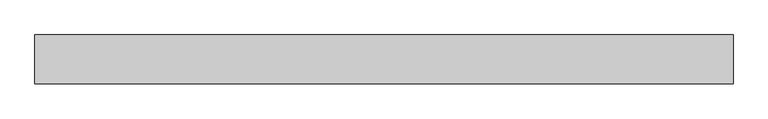
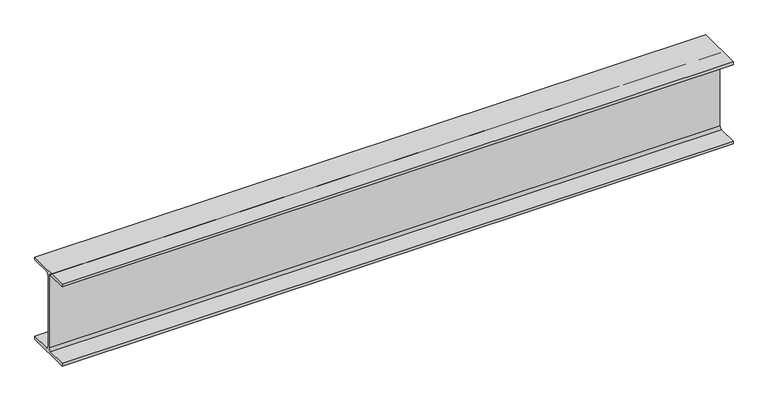
"""IFC4 building model written with IfcOpenShell, lengths in millimetres: beam geometry, Old_Steel Beam_H-KSD3502 : H_SB_ASB_H-200×200x8x12."""

import ifcopenshell
import ifcopenshell.guid

model = None  # the IFC model being written
_history = None  # IfcOwnerHistory: only IFC2X3 demands one
_inside = {}  # id of a spatial element -> (the spatial element, [elements in it])
_under = {}  # id of a project, library or spatial element -> (it, [spatial elements below it])
_declared = {}  # id of a project -> (the project, [libraries it declares])
_typed = {}  # id of a type object -> (the type object, [elements of that type])
_made_of = {}  # id of a material, layer set ... -> (it, [elements and type objects made of it])


def new_model(schema):
    """Start an empty IFC model of exactly this schema.

    Asked for "IFC4X3", IfcOpenShell would pick the latest addendum, in which some entities
    have other attributes; the version numbers below select the first issue.
    IFC2X3 requires an IfcOwnerHistory on every rooted entity: one is made here for all.
    """
    global model, _history
    if schema == "IFC4X3":
        model = ifcopenshell.file(schema_version=(4, 3, 0, 0))
    else:
        model = ifcopenshell.file(schema=schema)
    _inside.clear()
    _under.clear()
    _declared.clear()
    _typed.clear()
    _made_of.clear()
    _history = None
    if model.schema == "IFC2X3":
        org = make("IfcOrganization", Name="unknown")
        user = make(
            "IfcPersonAndOrganization",
            ThePerson=make("IfcPerson", FamilyName="unknown"),
            TheOrganization=org,
        )
        app = make(
            "IfcApplication",
            ApplicationDeveloper=org,
            Version="unknown",
            ApplicationFullName="unknown",
            ApplicationIdentifier="unknown",
        )
        _history = make(
            "IfcOwnerHistory",
            OwningUser=user,
            OwningApplication=app,
            ChangeAction="ADDED",
            CreationDate=0,
        )
    return model


def make(cls, **values):
    """One entity of the class cls with the attributes given. An attribute that is None is left unset."""
    return model.create_entity(
        cls, **{name: value for name, value in values.items() if value is not None}
    )


def rooted(cls, **values):
    """An entity with a GlobalId (a new one), such as an element, a storey or a relation."""
    return make(cls, GlobalId=ifcopenshell.guid.new(), OwnerHistory=_history, **values)


def si_unit(unit_type, name, prefix=None):
    """IfcSIUnit, for example si_unit("LENGTHUNIT", "METRE", prefix="MILLI")."""
    return make("IfcSIUnit", UnitType=unit_type, Prefix=prefix, Name=name)


def assignment(units):
    """IfcUnitAssignment: the units of a project."""
    return None if units is None else make("IfcUnitAssignment", Units=units)


def point(xyz):
    """IfcCartesianPoint."""
    return None if xyz is None else make("IfcCartesianPoint", Coordinates=xyz)


def direction(xyz):
    """IfcDirection."""
    return None if xyz is None else make("IfcDirection", DirectionRatios=xyz)


def frame(location, z_axis=None, x_axis=None):
    """IfcAxis2Placement3D, a coordinate frame: its origin and axes. An axis left out is left unset."""
    return make(
        "IfcAxis2Placement3D",
        Location=point(location),
        Axis=direction(z_axis),
        RefDirection=direction(x_axis),
    )


def frame_2d(location, x_axis=None):
    """IfcAxis2Placement2D, a coordinate frame in the plane: its origin and x axis."""
    return make(
        "IfcAxis2Placement2D", Location=point(location), RefDirection=direction(x_axis)
    )


def origin():
    """The frame at (0, 0, 0) with its axes left unset."""
    return frame((0.0, 0.0, 0.0))


def place(relative_to, where):
    """IfcLocalPlacement: puts the frame where relative to a parent placement (None: the world)."""
    return make(
        "IfcLocalPlacement", PlacementRelTo=relative_to, RelativePlacement=where
    )


def context(
    kind, dimensions, precision=None, world=None, true_north=None, identifier=None
):
    """IfcGeometricRepresentationContext, for example the 3D "Model" context."""
    return make(
        "IfcGeometricRepresentationContext",
        ContextIdentifier=identifier,
        ContextType=kind,
        CoordinateSpaceDimension=dimensions,
        Precision=precision,
        WorldCoordinateSystem=world,
        TrueNorth=true_north,
    )


def project(units=None, contexts=None):
    """IfcProject with its units and contexts."""
    return rooted(
        "IfcProject",
        Name="project",
        RepresentationContexts=contexts,
        UnitsInContext=assignment(units),
    )


def spatial(cls, under=None, at=None, **own):
    """A site, building, storey or space (cls), placed at a placement, below another one or the project."""
    s = rooted(cls, ObjectPlacement=at, **own)
    if under is not None:
        _under.setdefault(under.id(), (under, []))[1].append(s)
    return s


def polyline(points):
    """IfcPolyline through the points."""
    return make("IfcPolyline", Points=[point(p) for p in points])


def circle_curve(where, radius):
    """IfcCircle in the frame where."""
    return make("IfcCircle", Position=where, Radius=radius)


def trimmed(basis, trim1, trim2, sense, master):
    """IfcTrimmedCurve: the piece of a basis curve between two trims."""
    return make(
        "IfcTrimmedCurve",
        BasisCurve=basis,
        Trim1=trim1,
        Trim2=trim2,
        SenseAgreement=sense,
        MasterRepresentation=master,
    )


def segment(curve, same_sense, transition):
    """IfcCompositeCurveSegment."""
    return make(
        "IfcCompositeCurveSegment",
        Transition=transition,
        SameSense=same_sense,
        ParentCurve=curve,
    )


def composite_curve(segments, self_intersect=None):
    """IfcCompositeCurve: segments joined end to end."""
    return make("IfcCompositeCurve", Segments=segments, SelfIntersect=self_intersect)


def outline(outer, holes=None, kind="AREA"):
    """IfcArbitraryClosedProfileDef: a profile drawn as a closed curve; with holes, ...WithVoids."""
    if holes is None:
        return make("IfcArbitraryClosedProfileDef", ProfileType=kind, OuterCurve=outer)
    return make(
        "IfcArbitraryProfileDefWithVoids",
        ProfileType=kind,
        OuterCurve=outer,
        InnerCurves=holes,
    )


def extrude(swept, where, along, depth):
    """IfcExtrudedAreaSolid: the profile swept, set in the frame where, extruded along a direction by depth."""
    return make(
        "IfcExtrudedAreaSolid",
        SweptArea=swept,
        Position=where,
        ExtrudedDirection=direction(along),
        Depth=depth,
    )


def shape(context_of_items, identifier, shape_type, items):
    """IfcShapeRepresentation: the items that make up one representation, for example the "Body"."""
    return make(
        "IfcShapeRepresentation",
        ContextOfItems=context_of_items,
        RepresentationIdentifier=identifier,
        RepresentationType=shape_type,
        Items=items,
    )


def source(mapping_origin, context_of_items, identifier, shape_type, items):
    """IfcRepresentationMap: a shape defined once, which mapped items show again and again."""
    return make(
        "IfcRepresentationMap",
        MappingOrigin=mapping_origin,
        MappedRepresentation=shape(context_of_items, identifier, shape_type, items),
    )


def transform(
    local_origin,
    x_axis=None,
    y_axis=None,
    z_axis=None,
    scale=None,
    scale2=None,
    scale3=None,
    uniform=True,
):
    """IfcCartesianTransformationOperator3D, or its non-uniform kind. x_axis, y_axis, z_axis: its Axis1, 2, 3."""
    if uniform:
        return make(
            "IfcCartesianTransformationOperator3D",
            Axis1=direction(x_axis),
            Axis2=direction(y_axis),
            LocalOrigin=point(local_origin),
            Scale=scale,
            Axis3=direction(z_axis),
        )
    return make(
        "IfcCartesianTransformationOperator3DnonUniform",
        Axis1=direction(x_axis),
        Axis2=direction(y_axis),
        LocalOrigin=point(local_origin),
        Scale=scale,
        Axis3=direction(z_axis),
        Scale2=scale2,
        Scale3=scale3,
    )


def mapped(mapping_source, mapping_target):
    """IfcMappedItem: shows the shape of a source again, moved by a transform."""
    return make(
        "IfcMappedItem", MappingSource=mapping_source, MappingTarget=mapping_target
    )


def made_of(thing, what):
    """Note that an element or type object is made of a material, layer set ...; save() writes the relation."""
    if what is not None:
        _made_of.setdefault(what.id(), (what, []))[1].append(thing)
    return thing


def element(
    cls,
    number,
    at=None,
    inside=None,
    cuts=None,
    type_object=None,
    material=None,
    context=None,
    identifier="Body",
    shape_type=None,
    held_by="IfcProductDefinitionShape",
    body=None,
    shapes=None,
    **own,
):
    """One element of the class cls, such as IfcWall. Its Tag is "e" and its number.

    at: its placement. inside: the storey or other place that contains it. cuts: it is an
    opening in that element (IfcRelVoidsElement). A single representation is given by context,
    identifier, shape_type and body (its items); several are given by shapes. held_by: the class
    of the entity that holds the representations. save() writes the other relations.
    """
    e = rooted(cls, Tag="e%d" % number, ObjectPlacement=at, **own)
    if body is not None:
        shapes = [shape(context, identifier, shape_type, body)]
    if shapes is not None:
        e.Representation = make(held_by, Representations=shapes)
    if inside is not None:
        _inside.setdefault(inside.id(), (inside, []))[1].append(e)
    if cuts is not None:
        rooted(
            "IfcRelVoidsElement", RelatingBuildingElement=cuts, RelatedOpeningElement=e
        )
    if type_object is not None:
        _typed.setdefault(type_object.id(), (type_object, []))[1].append(e)
    return made_of(e, material)


def aggregate(whole, parts):
    """IfcRelAggregates: a whole, such as a stair, and the parts it consists of."""
    return rooted("IfcRelAggregates", RelatingObject=whole, RelatedObjects=parts)


def save(model, path):
    """Write the relations noted so far, then the file.

    IfcRelAggregates (storeys below a building ...), IfcRelContainedInSpatialStructure (elements
    in a storey), IfcRelDefinesByType, IfcRelAssociatesMaterial and IfcRelDeclares: one each for
    every whole, place, type object, material and project.
    """
    for whole, parts in _under.values():
        aggregate(whole, parts)
    for where, things in _inside.values():
        rooted(
            "IfcRelContainedInSpatialStructure",
            RelatedElements=things,
            RelatingStructure=where,
        )
    for kind, things in _typed.values():
        rooted("IfcRelDefinesByType", RelatedObjects=things, RelatingType=kind)
    for what, things in _made_of.values():
        rooted("IfcRelAssociatesMaterial", RelatedObjects=things, RelatingMaterial=what)
    for by, libraries in _declared.values():
        rooted("IfcRelDeclares", RelatingContext=by, RelatedDefinitions=libraries)
    model.write(path)


def beam_bc7b9760(model_context):
    return source(origin(), model_context, "Body", "SweptSolid", [
        extrude(outline(composite_curve([segment(polyline([(82.5, -141.5), (82.5, -151.7), (-82.5, -151.7), (-82.5, -141.5), (-11.9, -141.5)]), True, "CONTINUOUS"), segment(trimmed(circle_curve(frame_2d((-11.9, -132.6)), 8.9), [point((-11.9, -141.5))], [point((-3.0, -132.6))], True, "CARTESIAN"), True, "CONTINUOUS"), segment(polyline([(-3.0, -132.6), (-3.0, 132.6)]), True, "CONTINUOUS"), segment(trimmed(circle_curve(frame_2d((-11.9, 132.6)), 8.9), [point((-3.0, 132.6))], [point((-11.9, 141.5))], True, "CARTESIAN"), True, "CONTINUOUS"), segment(polyline([(-11.9, 141.5), (-82.5, 141.5), (-82.5, 151.7), (82.5, 151.7), (82.5, 141.5), (11.9, 141.5)]), True, "CONTINUOUS"), segment(trimmed(circle_curve(frame_2d((11.9, 132.6)), 8.9), [point((11.9, 141.5))], [point((3.0, 132.6))], True, "CARTESIAN"), True, "CONTINUOUS"), segment(polyline([(3.0, 132.6), (3.0, -132.6)]), True, "CONTINUOUS"), segment(trimmed(circle_curve(frame_2d((11.9, -132.6)), 8.9), [point((3.0, -132.6))], [point((11.9, -141.5))], True, "CARTESIAN"), True, "CONTINUOUS"), segment(polyline([(11.9, -141.5), (82.5, -141.5)]), True, "CONTINUOUS")], self_intersect=False)), frame((-1166.1355565, 0.0, 0.0), z_axis=(1.0, 0.0, 0.0), x_axis=(0.0, 1.0, 0.0)), (0.0, 0.0, 1.0), 2350.5623426),
    ])


if __name__ == "__main__":
    model = new_model("IFC4")
    model_context = context("Model", 3, world=origin())
    ifc_project = project(units=[si_unit("LENGTHUNIT", "METRE", prefix="MILLI")], contexts=[model_context])
    site = spatial("IfcSite", under=ifc_project)
    building = spatial("IfcBuilding", under=site)
    placement = place(None, origin())
    beam_shape = beam_bc7b9760(model_context)
    element("IfcBeam", 1, ObjectType="Old_Steel Beam_H-KSD3502 : H_SB_ASB_H-200×200x8x12", at=placement, inside=building, context=model_context, shape_type="MappedRepresentation", body=[
        mapped(beam_shape, transform((0.0, 0.0, 0.0), x_axis=(1.0, 0.0, 0.0), y_axis=(0.0, 1.0, 0.0), z_axis=(0.0, 0.0, 1.0))),
    ])
    save(model, "model.ifc")

# Revit data of these elements
# Type "Old_Steel Beam_H-KSD3502 : H_SB_ASB_H-200×200x8x12"
#   Width = 20.0 cm
#   Web Thickness = 0.8 cm
#   Web Fillet = 1.3 cm
#   Warping Constant = 141376.0 cm⁶
#   Torsional Moment of Inertia = 26.2485 cm⁴
#   Torsional Modulus = 1.0 cm³
#   Section Area = 63.53 cm²
#   Plastic Modulus weak axis = 244.0 cm³
#   Plastic Modulus strong axis = 525.0 cm³
#   Perimeter = 1.16 m²/m
#   Nominal Weight = 49.90 kgf/m
#   Moment of Inertia weak axis = 1600.00 cm⁴
#   Moment of Inertia strong axis = 4720.00 cm⁴
#   Height = 20.0 cm
#   Flange Thickness = 1.2 cm
#   Elastic Modulus weak axis = 160.0 cm³
#   Elastic Modulus strong axis = 472.0 cm³
#   Centroid Vertical = 10.0 cm
#   Centroid Horizontal = 10.0 cm
#   Length [instance default] = 1.5240 m
#   Structural Material [instance default] = Steel, 45-345
#   Assembly Code = ""
# Element 1 (IfcBeam, "Old_Steel Beam_H-KSD3502 : H_SB_ASB_H-200×200x8x12")
#   Structural Material = none
# Materials
#   "Steel, 45-345": class "Metal", colour RGB 189 187 185, transparency 0, Description = "Steel 345 MPa", Cost = 0
